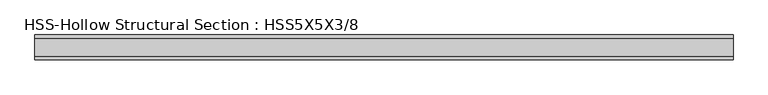
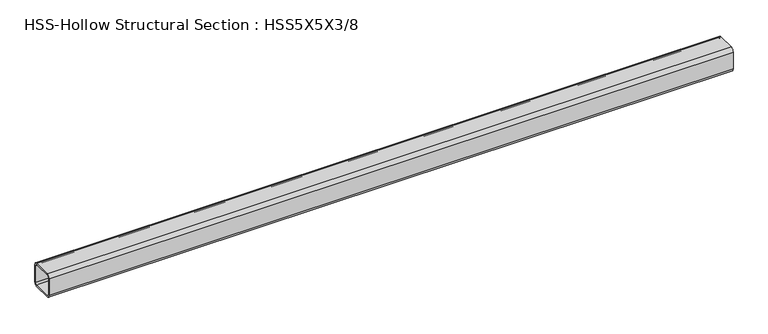
"""IFC4 building model written with IfcOpenShell, lengths in millimetres: member geometry, HSS-Hollow Structural Section : HSS5X5X3/8."""

import ifcopenshell
import ifcopenshell.guid

model = None  # the IFC model being written
_history = None  # IfcOwnerHistory: only IFC2X3 demands one
_inside = {}  # id of a spatial element -> (the spatial element, [elements in it])
_under = {}  # id of a project, library or spatial element -> (it, [spatial elements below it])
_declared = {}  # id of a project -> (the project, [libraries it declares])
_typed = {}  # id of a type object -> (the type object, [elements of that type])
_made_of = {}  # id of a material, layer set ... -> (it, [elements and type objects made of it])


def new_model(schema):
    """Start an empty IFC model of exactly this schema.

    Asked for "IFC4X3", IfcOpenShell would pick the latest addendum, in which some entities
    have other attributes; the version numbers below select the first issue.
    IFC2X3 requires an IfcOwnerHistory on every rooted entity: one is made here for all.
    """
    global model, _history
    if schema == "IFC4X3":
        model = ifcopenshell.file(schema_version=(4, 3, 0, 0))
    else:
        model = ifcopenshell.file(schema=schema)
    _inside.clear()
    _under.clear()
    _declared.clear()
    _typed.clear()
    _made_of.clear()
    _history = None
    if model.schema == "IFC2X3":
        org = make("IfcOrganization", Name="unknown")
        user = make(
            "IfcPersonAndOrganization",
            ThePerson=make("IfcPerson", FamilyName="unknown"),
            TheOrganization=org,
        )
        app = make(
            "IfcApplication",
            ApplicationDeveloper=org,
            Version="unknown",
            ApplicationFullName="unknown",
            ApplicationIdentifier="unknown",
        )
        _history = make(
            "IfcOwnerHistory",
            OwningUser=user,
            OwningApplication=app,
            ChangeAction="ADDED",
            CreationDate=0,
        )
    return model


def make(cls, **values):
    """One entity of the class cls with the attributes given. An attribute that is None is left unset."""
    return model.create_entity(
        cls, **{name: value for name, value in values.items() if value is not None}
    )


def rooted(cls, **values):
    """An entity with a GlobalId (a new one), such as an element, a storey or a relation."""
    return make(cls, GlobalId=ifcopenshell.guid.new(), OwnerHistory=_history, **values)


def si_unit(unit_type, name, prefix=None):
    """IfcSIUnit, for example si_unit("LENGTHUNIT", "METRE", prefix="MILLI")."""
    return make("IfcSIUnit", UnitType=unit_type, Prefix=prefix, Name=name)


def assignment(units):
    """IfcUnitAssignment: the units of a project."""
    return None if units is None else make("IfcUnitAssignment", Units=units)


def point(xyz):
    """IfcCartesianPoint."""
    return None if xyz is None else make("IfcCartesianPoint", Coordinates=xyz)


def direction(xyz):
    """IfcDirection."""
    return None if xyz is None else make("IfcDirection", DirectionRatios=xyz)


def frame(location, z_axis=None, x_axis=None):
    """IfcAxis2Placement3D, a coordinate frame: its origin and axes. An axis left out is left unset."""
    return make(
        "IfcAxis2Placement3D",
        Location=point(location),
        Axis=direction(z_axis),
        RefDirection=direction(x_axis),
    )


def frame_2d(location, x_axis=None):
    """IfcAxis2Placement2D, a coordinate frame in the plane: its origin and x axis."""
    return make(
        "IfcAxis2Placement2D", Location=point(location), RefDirection=direction(x_axis)
    )


def origin():
    """The frame at (0, 0, 0) with its axes left unset."""
    return frame((0.0, 0.0, 0.0))


def place(relative_to, where):
    """IfcLocalPlacement: puts the frame where relative to a parent placement (None: the world)."""
    return make(
        "IfcLocalPlacement", PlacementRelTo=relative_to, RelativePlacement=where
    )


def context(
    kind, dimensions, precision=None, world=None, true_north=None, identifier=None
):
    """IfcGeometricRepresentationContext, for example the 3D "Model" context."""
    return make(
        "IfcGeometricRepresentationContext",
        ContextIdentifier=identifier,
        ContextType=kind,
        CoordinateSpaceDimension=dimensions,
        Precision=precision,
        WorldCoordinateSystem=world,
        TrueNorth=true_north,
    )


def project(units=None, contexts=None):
    """IfcProject with its units and contexts."""
    return rooted(
        "IfcProject",
        Name="project",
        RepresentationContexts=contexts,
        UnitsInContext=assignment(units),
    )


def spatial(cls, under=None, at=None, **own):
    """A site, building, storey or space (cls), placed at a placement, below another one or the project."""
    s = rooted(cls, ObjectPlacement=at, **own)
    if under is not None:
        _under.setdefault(under.id(), (under, []))[1].append(s)
    return s


def polyline(points):
    """IfcPolyline through the points."""
    return make("IfcPolyline", Points=[point(p) for p in points])


def circle_curve(where, radius):
    """IfcCircle in the frame where."""
    return make("IfcCircle", Position=where, Radius=radius)


def trimmed(basis, trim1, trim2, sense, master):
    """IfcTrimmedCurve: the piece of a basis curve between two trims."""
    return make(
        "IfcTrimmedCurve",
        BasisCurve=basis,
        Trim1=trim1,
        Trim2=trim2,
        SenseAgreement=sense,
        MasterRepresentation=master,
    )


def segment(curve, same_sense, transition):
    """IfcCompositeCurveSegment."""
    return make(
        "IfcCompositeCurveSegment",
        Transition=transition,
        SameSense=same_sense,
        ParentCurve=curve,
    )


def composite_curve(segments, self_intersect=None):
    """IfcCompositeCurve: segments joined end to end."""
    return make("IfcCompositeCurve", Segments=segments, SelfIntersect=self_intersect)


def outline(outer, holes=None, kind="AREA"):
    """IfcArbitraryClosedProfileDef: a profile drawn as a closed curve; with holes, ...WithVoids."""
    if holes is None:
        return make("IfcArbitraryClosedProfileDef", ProfileType=kind, OuterCurve=outer)
    return make(
        "IfcArbitraryProfileDefWithVoids",
        ProfileType=kind,
        OuterCurve=outer,
        InnerCurves=holes,
    )


def extrude(swept, where, along, depth):
    """IfcExtrudedAreaSolid: the profile swept, set in the frame where, extruded along a direction by depth."""
    return make(
        "IfcExtrudedAreaSolid",
        SweptArea=swept,
        Position=where,
        ExtrudedDirection=direction(along),
        Depth=depth,
    )


def shape(context_of_items, identifier, shape_type, items):
    """IfcShapeRepresentation: the items that make up one representation, for example the "Body"."""
    return make(
        "IfcShapeRepresentation",
        ContextOfItems=context_of_items,
        RepresentationIdentifier=identifier,
        RepresentationType=shape_type,
        Items=items,
    )


def source(mapping_origin, context_of_items, identifier, shape_type, items):
    """IfcRepresentationMap: a shape defined once, which mapped items show again and again."""
    return make(
        "IfcRepresentationMap",
        MappingOrigin=mapping_origin,
        MappedRepresentation=shape(context_of_items, identifier, shape_type, items),
    )


def transform(
    local_origin,
    x_axis=None,
    y_axis=None,
    z_axis=None,
    scale=None,
    scale2=None,
    scale3=None,
    uniform=True,
):
    """IfcCartesianTransformationOperator3D, or its non-uniform kind. x_axis, y_axis, z_axis: its Axis1, 2, 3."""
    if uniform:
        return make(
            "IfcCartesianTransformationOperator3D",
            Axis1=direction(x_axis),
            Axis2=direction(y_axis),
            LocalOrigin=point(local_origin),
            Scale=scale,
            Axis3=direction(z_axis),
        )
    return make(
        "IfcCartesianTransformationOperator3DnonUniform",
        Axis1=direction(x_axis),
        Axis2=direction(y_axis),
        LocalOrigin=point(local_origin),
        Scale=scale,
        Axis3=direction(z_axis),
        Scale2=scale2,
        Scale3=scale3,
    )


def mapped(mapping_source, mapping_target):
    """IfcMappedItem: shows the shape of a source again, moved by a transform."""
    return make(
        "IfcMappedItem", MappingSource=mapping_source, MappingTarget=mapping_target
    )


def made_of(thing, what):
    """Note that an element or type object is made of a material, layer set ...; save() writes the relation."""
    if what is not None:
        _made_of.setdefault(what.id(), (what, []))[1].append(thing)
    return thing


def element(
    cls,
    number,
    at=None,
    inside=None,
    cuts=None,
    type_object=None,
    material=None,
    context=None,
    identifier="Body",
    shape_type=None,
    held_by="IfcProductDefinitionShape",
    body=None,
    shapes=None,
    **own,
):
    """One element of the class cls, such as IfcWall. Its Tag is "e" and its number.

    at: its placement. inside: the storey or other place that contains it. cuts: it is an
    opening in that element (IfcRelVoidsElement). A single representation is given by context,
    identifier, shape_type and body (its items); several are given by shapes. held_by: the class
    of the entity that holds the representations. save() writes the other relations.
    """
    e = rooted(cls, Tag="e%d" % number, ObjectPlacement=at, **own)
    if body is not None:
        shapes = [shape(context, identifier, shape_type, body)]
    if shapes is not None:
        e.Representation = make(held_by, Representations=shapes)
    if inside is not None:
        _inside.setdefault(inside.id(), (inside, []))[1].append(e)
    if cuts is not None:
        rooted(
            "IfcRelVoidsElement", RelatingBuildingElement=cuts, RelatedOpeningElement=e
        )
    if type_object is not None:
        _typed.setdefault(type_object.id(), (type_object, []))[1].append(e)
    return made_of(e, material)


def aggregate(whole, parts):
    """IfcRelAggregates: a whole, such as a stair, and the parts it consists of."""
    return rooted("IfcRelAggregates", RelatingObject=whole, RelatedObjects=parts)


def save(model, path):
    """Write the relations noted so far, then the file.

    IfcRelAggregates (storeys below a building ...), IfcRelContainedInSpatialStructure (elements
    in a storey), IfcRelDefinesByType, IfcRelAssociatesMaterial and IfcRelDeclares: one each for
    every whole, place, type object, material and project.
    """
    for whole, parts in _under.values():
        aggregate(whole, parts)
    for where, things in _inside.values():
        rooted(
            "IfcRelContainedInSpatialStructure",
            RelatedElements=things,
            RelatingStructure=where,
        )
    for kind, things in _typed.values():
        rooted("IfcRelDefinesByType", RelatedObjects=things, RelatingType=kind)
    for what, things in _made_of.values():
        rooted("IfcRelAssociatesMaterial", RelatedObjects=things, RelatingMaterial=what)
    for by, libraries in _declared.values():
        rooted("IfcRelDeclares", RelatingContext=by, RelatedDefinitions=libraries)
    model.write(path)


def hss_hollow_structural_section_hss5x5x3_8_98c1edb9(model_context):
    return source(origin(), model_context, "Body", "SweptSolid", [
        extrude(outline(composite_curve([segment(polyline([(63.5, 45.7708), (63.5, -45.7708)]), True, "CONTINUOUS"), segment(trimmed(circle_curve(frame_2d((45.7708, -45.7708)), 17.7292), [point((63.5, -45.7708))], [point((45.7708, -63.5))], False, "CARTESIAN"), True, "CONTINUOUS"), segment(polyline([(45.7708, -63.5), (-45.7708, -63.5)]), True, "CONTINUOUS"), segment(trimmed(circle_curve(frame_2d((-45.7708, -45.7708)), 17.7292), [point((-45.7708, -63.5))], [point((-63.5, -45.7708))], False, "CARTESIAN"), True, "CONTINUOUS"), segment(polyline([(-63.5, -45.7708), (-63.5, 45.7708)]), True, "CONTINUOUS"), segment(trimmed(circle_curve(frame_2d((-45.7708, 45.7708)), 17.7292), [point((-63.5, 45.7708))], [point((-45.7708, 63.5))], False, "CARTESIAN"), True, "CONTINUOUS"), segment(polyline([(-45.7708, 63.5), (45.7708, 63.5)]), True, "CONTINUOUS"), segment(trimmed(circle_curve(frame_2d((45.7708, 45.7708)), 17.7292), [point((45.7708, 63.5))], [point((63.5, 45.7708))], False, "CARTESIAN"), True, "CONTINUOUS")], self_intersect=False), holes=[composite_curve([segment(trimmed(circle_curve(frame_2d((-45.7708, 45.7708)), 8.8646), [point((-45.7708, 54.6354))], [point((-54.6354, 45.7708))], True, "CARTESIAN"), True, "CONTINUOUS"), segment(polyline([(-54.6354, 45.7708), (-54.6354, -45.7708)]), True, "CONTINUOUS"), segment(trimmed(circle_curve(frame_2d((-45.7708, -45.7708)), 8.8646), [point((-54.6354, -45.7708))], [point((-45.7708, -54.6354))], True, "CARTESIAN"), True, "CONTINUOUS"), segment(polyline([(-45.7708, -54.6354), (45.7708, -54.6354)]), True, "CONTINUOUS"), segment(trimmed(circle_curve(frame_2d((45.7708, -45.7708)), 8.8646), [point((45.7708, -54.6354))], [point((54.6354, -45.7708))], True, "CARTESIAN"), True, "CONTINUOUS"), segment(polyline([(54.6354, -45.7708), (54.6354, 45.7708)]), True, "CONTINUOUS"), segment(trimmed(circle_curve(frame_2d((45.7708, 45.7708)), 8.8646), [point((54.6354, 45.7708))], [point((45.7708, 54.6354))], True, "CARTESIAN"), True, "CONTINUOUS"), segment(polyline([(45.7708, 54.6354), (-45.7708, 54.6354)]), True, "CONTINUOUS")], self_intersect=False)]), frame((-1774.2408481, 0.0, 0.0), z_axis=(1.0, 0.0, 0.0), x_axis=(0.0, 1.0, 0.0)), (0.0, 0.0, 1.0), 3548.4816962),
    ])


if __name__ == "__main__":
    model = new_model("IFC4")
    model_context = context("Model", 3, world=origin())
    ifc_project = project(units=[si_unit("LENGTHUNIT", "METRE", prefix="MILLI")], contexts=[model_context])
    site = spatial("IfcSite", under=ifc_project)
    building = spatial("IfcBuilding", under=site)
    placement = place(None, origin())
    hss_hollow_structural_section_hss5x5x3_8_shape = hss_hollow_structural_section_hss5x5x3_8_98c1edb9(model_context)
    element("IfcMember", 1, ObjectType="HSS-Hollow Structural Section : HSS5X5X3/8", at=placement, inside=building, context=model_context, shape_type="MappedRepresentation", body=[
        mapped(hss_hollow_structural_section_hss5x5x3_8_shape, transform((0.0, 0.0, 0.0), x_axis=(1.0, 0.0, 0.0), y_axis=(0.0, 1.0, 0.0), z_axis=(0.0, 0.0, 1.0))),
    ])
    save(model, "model.ifc")

# Revit data of these elements
# Type "HSS-Hollow Structural Section : HSS5X5X3/8"
#   Assembly Code = "B10"
#   Shape = "Square"
#   W = 22.3
#   Ht = 0' - 5"
#   Length [instance default] = 5' - 0"
#   b = 0' - 5"
#   kr = 0' - 0.698"
#   t = 0' - 0.349"
#   A = 0.0429167 SF
#   Structural Material [instance default] = Steel ASTM A500, Grade B, Rectangular and Square
# Element 1 (IfcMember, "HSS-Hollow Structural Section : HSS5X5X3/8")
#   Materials on its faces: "Steel ASTM A500, Grade B, Rectangular and Square"
# Materials
#   "Steel ASTM A500, Grade B, Rectangular and Square": class "Metal", colour RGB 199 199 199, transparency 0, Description = "Carbon steel", Cost = 0
